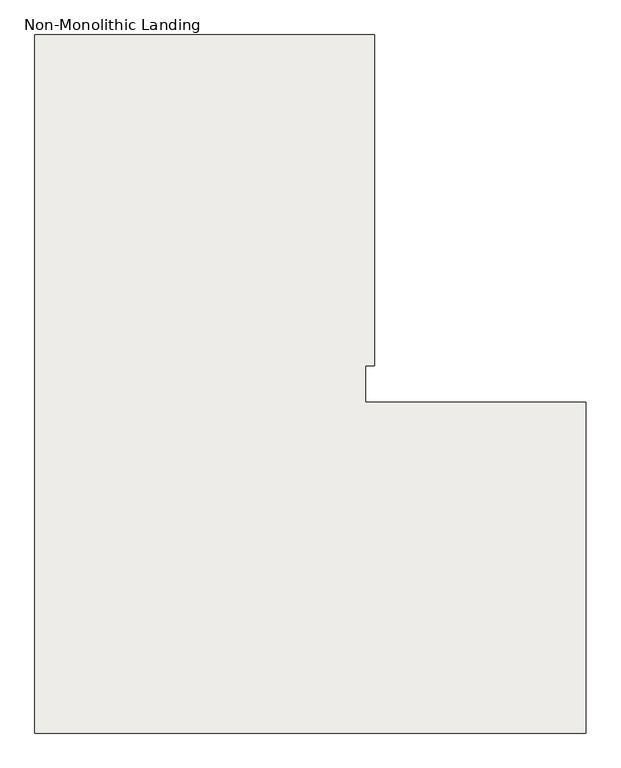
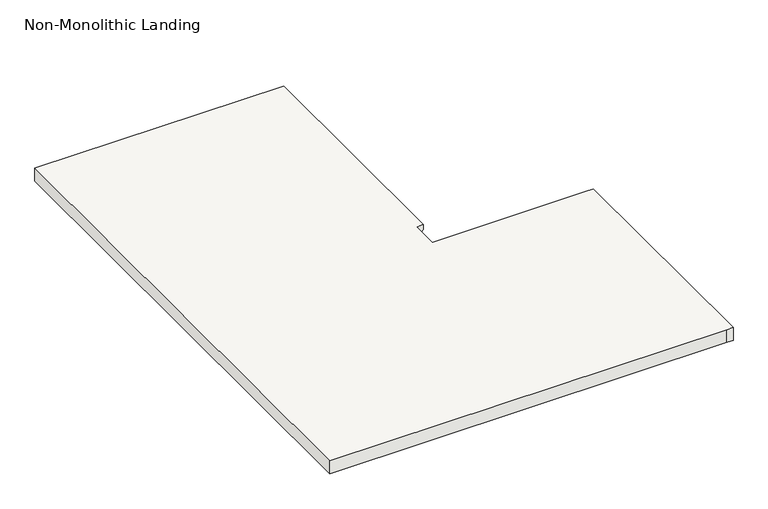
"""IFC4 building model written with IfcOpenShell, lengths in millimetres: slab geometry, Non-Monolithic Landing."""

from ifc_helpers import new_model, si_unit, origin, place, context, project, spatial, faceted_brep, source, transform, mapped, element, save


def non_monolithic_landing_6af57908(model_context):
    return source(origin(), model_context, "Body", "Brep", [
        faceted_brep([(24614.1840778, 26878.6156612, 265366.5), (24614.1840778, 26878.6156612, 265385.55), (24588.7840778, 26878.6156612, 265385.55), (24588.7840778, 26878.6156612, 265341.1), (24614.1840778, 27793.0156612, 265366.5), (24614.1840778, 27793.0156612, 265385.55), (24588.7840778, 27793.0156612, 265341.1), (23674.3840778, 27793.0156612, 265385.55), (23674.3840778, 25862.6156612, 265385.55), (25172.9840778, 25862.6156612, 265385.55), (25198.3840778, 25862.6156612, 265385.55), (25198.3840778, 26777.0156612, 265385.55), (25172.9840778, 26777.0156612, 265385.55), (24588.7840778, 26777.0156612, 265385.55), (24588.7840778, 27793.0156612, 265334.75), (24588.7840778, 26878.6156612, 265334.75), (24588.7840778, 26777.0156612, 265334.75), (25172.9840778, 26777.0156612, 265334.75), (25198.3840778, 26777.0156612, 265334.75), (25198.3840778, 25862.6156612, 265334.75), (25172.9840778, 25862.6156612, 265334.75), (23674.3840778, 25862.6156612, 265334.75), (23674.3840778, 27793.0156612, 265334.75)], [[[0, 1, 2, 3]], [[4, 5, 1, 0]], [[6, 4, 0, 3]], [[7, 8, 9, 10, 11, 12, 13, 2, 1, 5]], [[14, 15, 16, 17, 18, 19, 20, 21, 22]], [[15, 14, 6, 3]], [[2, 13, 16, 15, 3]], [[9, 8, 21, 20]], [[8, 7, 22, 21]], [[7, 5, 4, 6, 14, 22]], [[10, 9, 20, 19]], [[12, 11, 18, 17]], [[11, 10, 19, 18]], [[13, 12, 17, 16]]]),
    ])


if __name__ == "__main__":
    model = new_model("IFC4")
    model_context = context("Model", 3, world=origin())
    ifc_project = project(units=[si_unit("LENGTHUNIT", "METRE", prefix="MILLI")], contexts=[model_context])
    site = spatial("IfcSite", under=ifc_project)
    building = spatial("IfcBuilding", under=site)
    placement = place(None, origin())
    non_monolithic_landing_shape = non_monolithic_landing_6af57908(model_context)
    element("IfcSlab", 1, ObjectType="Non-Monolithic Landing", at=placement, inside=building, context=model_context, shape_type="MappedRepresentation", body=[
        mapped(non_monolithic_landing_shape, transform((0.0, 0.0, 0.0), x_axis=(1.0, 0.0, 0.0), y_axis=(0.0, 1.0, 0.0), z_axis=(0.0, 0.0, 1.0))),
    ])
    save(model, "model.ifc")

# Revit data of these elements
# Element 1 (IfcSlab, "Non-Monolithic Landing")
#   Materials on its faces: "SLOTTED WOOD FENCE (THERMALLY MODIFIED WOOD: ARBOR WOOD)\n(EXTERIOR STAIN : PENOFIN VERDE EXT. STAIN - COLOR: CEDAR)"
# Materials
#   "SLOTTED WOOD FENCE (THERMALLY MODIFIED WOOD: ARBOR WOOD)\n(EXTERIOR STAIN : PENOFIN VERDE EXT. STAIN - COLOR: CEDAR)": class "Wood", colour RGB 164 134 123, transparency 0, Description = "Pinus Echinata", Cost = 0
